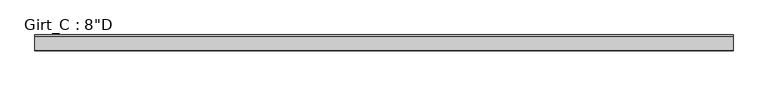
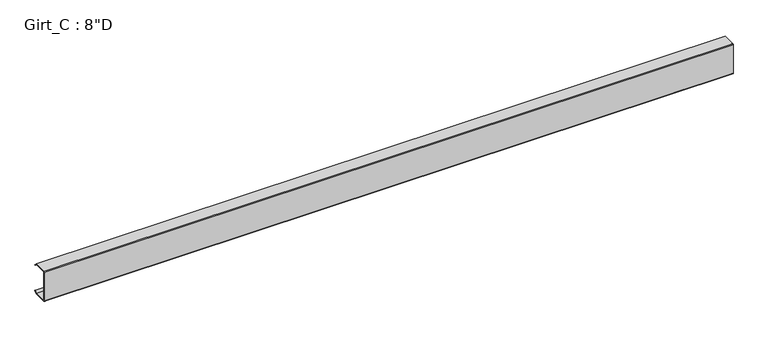
"""IFC4 building model written with IfcOpenShell, lengths in millimetres: beam geometry."""

import ifcopenshell
import ifcopenshell.guid

model = None  # the IFC model being written
_history = None  # IfcOwnerHistory: only IFC2X3 demands one
_inside = {}  # id of a spatial element -> (the spatial element, [elements in it])
_under = {}  # id of a project, library or spatial element -> (it, [spatial elements below it])
_declared = {}  # id of a project -> (the project, [libraries it declares])
_typed = {}  # id of a type object -> (the type object, [elements of that type])
_made_of = {}  # id of a material, layer set ... -> (it, [elements and type objects made of it])


def new_model(schema):
    """Start an empty IFC model of exactly this schema.

    Asked for "IFC4X3", IfcOpenShell would pick the latest addendum, in which some entities
    have other attributes; the version numbers below select the first issue.
    IFC2X3 requires an IfcOwnerHistory on every rooted entity: one is made here for all.
    """
    global model, _history
    if schema == "IFC4X3":
        model = ifcopenshell.file(schema_version=(4, 3, 0, 0))
    else:
        model = ifcopenshell.file(schema=schema)
    _inside.clear()
    _under.clear()
    _declared.clear()
    _typed.clear()
    _made_of.clear()
    _history = None
    if model.schema == "IFC2X3":
        org = make("IfcOrganization", Name="unknown")
        user = make(
            "IfcPersonAndOrganization",
            ThePerson=make("IfcPerson", FamilyName="unknown"),
            TheOrganization=org,
        )
        app = make(
            "IfcApplication",
            ApplicationDeveloper=org,
            Version="unknown",
            ApplicationFullName="unknown",
            ApplicationIdentifier="unknown",
        )
        _history = make(
            "IfcOwnerHistory",
            OwningUser=user,
            OwningApplication=app,
            ChangeAction="ADDED",
            CreationDate=0,
        )
    return model


def make(cls, **values):
    """One entity of the class cls with the attributes given. An attribute that is None is left unset."""
    return model.create_entity(
        cls, **{name: value for name, value in values.items() if value is not None}
    )


def rooted(cls, **values):
    """An entity with a GlobalId (a new one), such as an element, a storey or a relation."""
    return make(cls, GlobalId=ifcopenshell.guid.new(), OwnerHistory=_history, **values)


def si_unit(unit_type, name, prefix=None):
    """IfcSIUnit, for example si_unit("LENGTHUNIT", "METRE", prefix="MILLI")."""
    return make("IfcSIUnit", UnitType=unit_type, Prefix=prefix, Name=name)


def assignment(units):
    """IfcUnitAssignment: the units of a project."""
    return None if units is None else make("IfcUnitAssignment", Units=units)


def point(xyz):
    """IfcCartesianPoint."""
    return None if xyz is None else make("IfcCartesianPoint", Coordinates=xyz)


def direction(xyz):
    """IfcDirection."""
    return None if xyz is None else make("IfcDirection", DirectionRatios=xyz)


def frame(location, z_axis=None, x_axis=None):
    """IfcAxis2Placement3D, a coordinate frame: its origin and axes. An axis left out is left unset."""
    return make(
        "IfcAxis2Placement3D",
        Location=point(location),
        Axis=direction(z_axis),
        RefDirection=direction(x_axis),
    )


def frame_2d(location, x_axis=None):
    """IfcAxis2Placement2D, a coordinate frame in the plane: its origin and x axis."""
    return make(
        "IfcAxis2Placement2D", Location=point(location), RefDirection=direction(x_axis)
    )


def origin():
    """The frame at (0, 0, 0) with its axes left unset."""
    return frame((0.0, 0.0, 0.0))


def place(relative_to, where):
    """IfcLocalPlacement: puts the frame where relative to a parent placement (None: the world)."""
    return make(
        "IfcLocalPlacement", PlacementRelTo=relative_to, RelativePlacement=where
    )


def context(
    kind, dimensions, precision=None, world=None, true_north=None, identifier=None
):
    """IfcGeometricRepresentationContext, for example the 3D "Model" context."""
    return make(
        "IfcGeometricRepresentationContext",
        ContextIdentifier=identifier,
        ContextType=kind,
        CoordinateSpaceDimension=dimensions,
        Precision=precision,
        WorldCoordinateSystem=world,
        TrueNorth=true_north,
    )


def project(units=None, contexts=None):
    """IfcProject with its units and contexts."""
    return rooted(
        "IfcProject",
        Name="project",
        RepresentationContexts=contexts,
        UnitsInContext=assignment(units),
    )


def spatial(cls, under=None, at=None, **own):
    """A site, building, storey or space (cls), placed at a placement, below another one or the project."""
    s = rooted(cls, ObjectPlacement=at, **own)
    if under is not None:
        _under.setdefault(under.id(), (under, []))[1].append(s)
    return s


def polyline(points):
    """IfcPolyline through the points."""
    return make("IfcPolyline", Points=[point(p) for p in points])


def circle_curve(where, radius):
    """IfcCircle in the frame where."""
    return make("IfcCircle", Position=where, Radius=radius)


def trimmed(basis, trim1, trim2, sense, master):
    """IfcTrimmedCurve: the piece of a basis curve between two trims."""
    return make(
        "IfcTrimmedCurve",
        BasisCurve=basis,
        Trim1=trim1,
        Trim2=trim2,
        SenseAgreement=sense,
        MasterRepresentation=master,
    )


def segment(curve, same_sense, transition):
    """IfcCompositeCurveSegment."""
    return make(
        "IfcCompositeCurveSegment",
        Transition=transition,
        SameSense=same_sense,
        ParentCurve=curve,
    )


def composite_curve(segments, self_intersect=None):
    """IfcCompositeCurve: segments joined end to end."""
    return make("IfcCompositeCurve", Segments=segments, SelfIntersect=self_intersect)


def outline(outer, holes=None, kind="AREA"):
    """IfcArbitraryClosedProfileDef: a profile drawn as a closed curve; with holes, ...WithVoids."""
    if holes is None:
        return make("IfcArbitraryClosedProfileDef", ProfileType=kind, OuterCurve=outer)
    return make(
        "IfcArbitraryProfileDefWithVoids",
        ProfileType=kind,
        OuterCurve=outer,
        InnerCurves=holes,
    )


def extrude(swept, where, along, depth):
    """IfcExtrudedAreaSolid: the profile swept, set in the frame where, extruded along a direction by depth."""
    return make(
        "IfcExtrudedAreaSolid",
        SweptArea=swept,
        Position=where,
        ExtrudedDirection=direction(along),
        Depth=depth,
    )


def shape(context_of_items, identifier, shape_type, items):
    """IfcShapeRepresentation: the items that make up one representation, for example the "Body"."""
    return make(
        "IfcShapeRepresentation",
        ContextOfItems=context_of_items,
        RepresentationIdentifier=identifier,
        RepresentationType=shape_type,
        Items=items,
    )


def source(mapping_origin, context_of_items, identifier, shape_type, items):
    """IfcRepresentationMap: a shape defined once, which mapped items show again and again."""
    return make(
        "IfcRepresentationMap",
        MappingOrigin=mapping_origin,
        MappedRepresentation=shape(context_of_items, identifier, shape_type, items),
    )


def transform(
    local_origin,
    x_axis=None,
    y_axis=None,
    z_axis=None,
    scale=None,
    scale2=None,
    scale3=None,
    uniform=True,
):
    """IfcCartesianTransformationOperator3D, or its non-uniform kind. x_axis, y_axis, z_axis: its Axis1, 2, 3."""
    if uniform:
        return make(
            "IfcCartesianTransformationOperator3D",
            Axis1=direction(x_axis),
            Axis2=direction(y_axis),
            LocalOrigin=point(local_origin),
            Scale=scale,
            Axis3=direction(z_axis),
        )
    return make(
        "IfcCartesianTransformationOperator3DnonUniform",
        Axis1=direction(x_axis),
        Axis2=direction(y_axis),
        LocalOrigin=point(local_origin),
        Scale=scale,
        Axis3=direction(z_axis),
        Scale2=scale2,
        Scale3=scale3,
    )


def mapped(mapping_source, mapping_target):
    """IfcMappedItem: shows the shape of a source again, moved by a transform."""
    return make(
        "IfcMappedItem", MappingSource=mapping_source, MappingTarget=mapping_target
    )


def made_of(thing, what):
    """Note that an element or type object is made of a material, layer set ...; save() writes the relation."""
    if what is not None:
        _made_of.setdefault(what.id(), (what, []))[1].append(thing)
    return thing


def element(
    cls,
    number,
    at=None,
    inside=None,
    cuts=None,
    type_object=None,
    material=None,
    context=None,
    identifier="Body",
    shape_type=None,
    held_by="IfcProductDefinitionShape",
    body=None,
    shapes=None,
    **own,
):
    """One element of the class cls, such as IfcWall. Its Tag is "e" and its number.

    at: its placement. inside: the storey or other place that contains it. cuts: it is an
    opening in that element (IfcRelVoidsElement). A single representation is given by context,
    identifier, shape_type and body (its items); several are given by shapes. held_by: the class
    of the entity that holds the representations. save() writes the other relations.
    """
    e = rooted(cls, Tag="e%d" % number, ObjectPlacement=at, **own)
    if body is not None:
        shapes = [shape(context, identifier, shape_type, body)]
    if shapes is not None:
        e.Representation = make(held_by, Representations=shapes)
    if inside is not None:
        _inside.setdefault(inside.id(), (inside, []))[1].append(e)
    if cuts is not None:
        rooted(
            "IfcRelVoidsElement", RelatingBuildingElement=cuts, RelatedOpeningElement=e
        )
    if type_object is not None:
        _typed.setdefault(type_object.id(), (type_object, []))[1].append(e)
    return made_of(e, material)


def aggregate(whole, parts):
    """IfcRelAggregates: a whole, such as a stair, and the parts it consists of."""
    return rooted("IfcRelAggregates", RelatingObject=whole, RelatedObjects=parts)


def save(model, path):
    """Write the relations noted so far, then the file.

    IfcRelAggregates (storeys below a building ...), IfcRelContainedInSpatialStructure (elements
    in a storey), IfcRelDefinesByType, IfcRelAssociatesMaterial and IfcRelDeclares: one each for
    every whole, place, type object, material and project.
    """
    for whole, parts in _under.values():
        aggregate(whole, parts)
    for where, things in _inside.values():
        rooted(
            "IfcRelContainedInSpatialStructure",
            RelatedElements=things,
            RelatingStructure=where,
        )
    for kind, things in _typed.values():
        rooted("IfcRelDefinesByType", RelatedObjects=things, RelatingType=kind)
    for what, things in _made_of.values():
        rooted("IfcRelAssociatesMaterial", RelatedObjects=things, RelatingMaterial=what)
    for by, libraries in _declared.values():
        rooted("IfcRelDeclares", RelatingContext=by, RelatedDefinitions=libraries)
    model.write(path)


def beam_a20b00b4(model_context):
    return source(origin(), model_context, "Body", "SweptSolid", [
        extrude(outline(composite_curve([segment(polyline([(87.5109375, 101.6), (99.7560415, 87.0068534), (97.6278742, 85.221109), (86.2154765, 98.821875), (3.3005807, 98.821875)]), True, "CONTINUOUS"), segment(trimmed(circle_curve(frame_2d((3.3741066, 96.8381931)), 1.9850441), [point((3.3005807, 98.821875))], [point((1.3890625, 96.8381931))], True, "CARTESIAN"), True, "CONTINUOUS"), segment(polyline([(1.3890625, 96.8381931), (1.3890625, -96.8389339)]), True, "CONTINUOUS"), segment(trimmed(circle_curve(frame_2d((3.3748024, -96.8389339)), 1.9857399), [point((1.3890625, -96.8389339))], [point((3.2694106, -98.821875))], True, "CARTESIAN"), True, "CONTINUOUS"), segment(polyline([(3.2694106, -98.821875), (86.2154765, -98.821875), (97.6510975, -85.1934327), (99.7792647, -86.979177), (87.5109375, -101.6), (3.3734375, -101.6)]), True, "CONTINUOUS"), segment(trimmed(circle_curve(frame_2d((3.3734375, -96.8375)), 4.7625), [point((3.3734375, -101.6))], [point((-1.3890625, -96.8375))], False, "CARTESIAN"), True, "CONTINUOUS"), segment(polyline([(-1.3890625, -96.8375), (-1.3890625, 96.8375)]), True, "CONTINUOUS"), segment(trimmed(circle_curve(frame_2d((3.3734375, 96.8375)), 4.7625), [point((-1.3890625, 96.8375))], [point((3.3734375, 101.6))], False, "CARTESIAN"), True, "CONTINUOUS"), segment(polyline([(3.3734375, 101.6), (87.5109375, 101.6)]), True, "CONTINUOUS")], self_intersect=False)), frame((-2205.0375, 0.0, 0.0), z_axis=(1.0, 0.0, 0.0), x_axis=(0.0, 1.0, 0.0)), (0.0, 0.0, 1.0), 4410.075),
    ])


if __name__ == "__main__":
    model = new_model("IFC4")
    model_context = context("Model", 3, world=origin())
    ifc_project = project(units=[si_unit("LENGTHUNIT", "METRE", prefix="MILLI")], contexts=[model_context])
    site = spatial("IfcSite", under=ifc_project)
    building = spatial("IfcBuilding", under=site)
    placement = place(None, origin())
    beam_shape = beam_a20b00b4(model_context)
    element("IfcBeam", 1, ObjectType="Girt_C : 8\"D", at=placement, inside=building, context=model_context, shape_type="MappedRepresentation", body=[
        mapped(beam_shape, transform((0.0, 0.0, 0.0), x_axis=(1.0, 0.0, 0.0), y_axis=(0.0, 1.0, 0.0), z_axis=(0.0, 0.0, 1.0))),
    ])
    save(model, "model.ifc")

# Revit data of these elements
# Type "Girt_C : 8\"D"
#   half leg = 0' - 1 3/4"
#   Web_Thickness = 0' - 0 7/64"
#   Length [instance default] = 10' - 0"
#   Leg_1 = 0' - 3 1/2"
#   Height = 0' - 8"
#   Structural Material [instance default] = none
# Element 1 (IfcBeam, "Girt_C : 8\"D")
#   Structural Material = GALVANIZED 'CEE' SECTION (8.0x3.5C - SEE STRUCT. DWGS)
#   Materials on its faces: "GALVANIZED 'CEE' SECTION (8.0x3.5C - SEE STRUCT. DWGS)"
# Materials
#   "GALVANIZED 'CEE' SECTION (8.0x3.5C - SEE STRUCT. DWGS)": class "Metal", colour RGB 137 146 153, transparency 0, Description = "Steel, mill finish", Cost = 0
